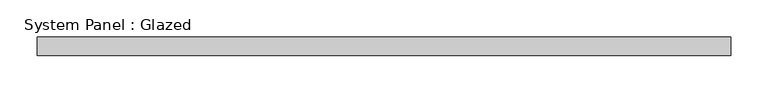
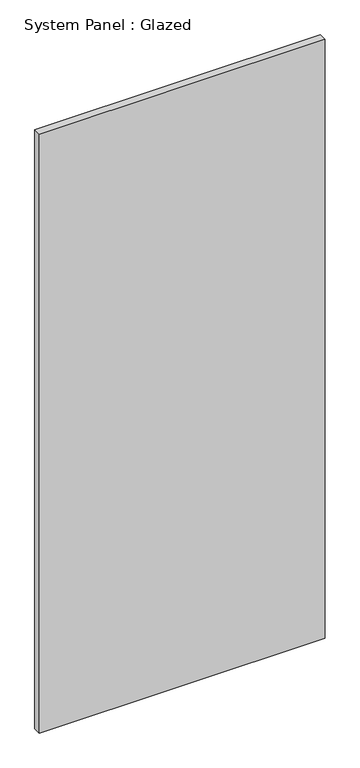
"""IFC4 building model written with IfcOpenShell, lengths in millimetres: plate geometry, System Panel : Glazed."""

from ifc_helpers import new_model, si_unit, origin, origin_with_axes, place, context, project, spatial, polyline, outline, extrude, source, transform, mapped, element, save


def system_panel_glazed_4c7b465e(model_context):
    return source(origin(), model_context, "Body", "SweptSolid", [
        extrude(outline(polyline([(467.5, 24.5), (-467.5, 24.5), (-467.5, 49.5), (467.5, 49.5), (467.5, 24.5)])), origin_with_axes(), (0.0, 0.0, 1.0), 2070.0),
    ])


if __name__ == "__main__":
    model = new_model("IFC4")
    model_context = context("Model", 3, world=origin())
    ifc_project = project(units=[si_unit("LENGTHUNIT", "METRE", prefix="MILLI")], contexts=[model_context])
    site = spatial("IfcSite", under=ifc_project)
    building = spatial("IfcBuilding", under=site)
    placement = place(None, origin())
    system_panel_glazed_shape = system_panel_glazed_4c7b465e(model_context)
    element("IfcPlate", 1, ObjectType="System Panel : Glazed", at=placement, inside=building, context=model_context, shape_type="MappedRepresentation", body=[
        mapped(system_panel_glazed_shape, transform((0.0, 0.0, 0.0), x_axis=(1.0, 0.0, 0.0), y_axis=(0.0, 1.0, 0.0), z_axis=(0.0, 0.0, 1.0))),
    ])
    save(model, "model.ifc")

# Revit data of these elements
# Type "System Panel : Glazed"
#   Construction Type Id = "GSP4R"
#   Analytic Construction = "1/8 in Pilkington single glazing"
#   Visual Light Transmittance = 0.9
#   Solar Heat Gain Coefficient = 0.86
#   Heat Transfer Coefficient (U) = 6.7069 W/(m²·K)
#   Define Thermal Properties by = 1
# Element 1 (IfcPlate, "System Panel : Glazed")
#   Materials on its faces: "Glass"
# Materials
#   "Glass": class "Glass", colour RGB 245 245 243, transparency 1, Description = "Soda Lime Glass", Cost = 0
